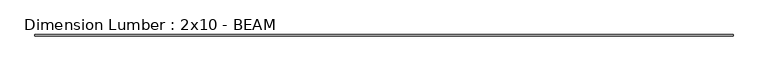
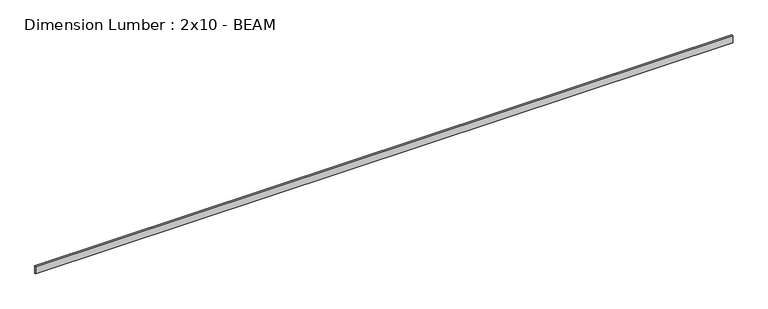
"""IFC4 building model written with IfcOpenShell, lengths in millimetres: beam geometry, Dimension Lumber : 2x10 - BEAM."""

from ifc_helpers import new_model, si_unit, frame, origin, place, context, project, spatial, polyline, outline, extrude, source, transform, mapped, element, save


def dimension_lumber_2x10_beam_73725c05(model_context):
    return source(origin(), model_context, "Body", "SweptSolid", [
        extrude(outline(polyline([(10626.7994141, 19.05), (10626.7994141, -19.05), (-10626.7994141, -19.05), (-10626.7994141, 19.05), (10626.7994141, 19.05)])), frame((0.0, 0.0, -117.475), z_axis=(0.0, 0.0, 1.0), x_axis=(1.0, 0.0, 0.0)), (0.0, 0.0, 1.0), 234.95),
    ])


if __name__ == "__main__":
    model = new_model("IFC4")
    model_context = context("Model", 3, world=origin())
    ifc_project = project(units=[si_unit("LENGTHUNIT", "METRE", prefix="MILLI")], contexts=[model_context])
    site = spatial("IfcSite", under=ifc_project)
    building = spatial("IfcBuilding", under=site)
    placement = place(None, origin())
    dimension_lumber_2x10_beam_shape = dimension_lumber_2x10_beam_73725c05(model_context)
    element("IfcBeam", 1, ObjectType="Dimension Lumber : 2x10 - BEAM", at=placement, inside=building, context=model_context, shape_type="MappedRepresentation", body=[
        mapped(dimension_lumber_2x10_beam_shape, transform((0.0, 0.0, 0.0), x_axis=(1.0, 0.0, 0.0), y_axis=(0.0, 1.0, 0.0), z_axis=(0.0, 0.0, 1.0))),
    ])
    save(model, "model.ifc")

# Revit data of these elements
# Type "Dimension Lumber : 2x10 - BEAM"
#   Assembly Code = "B10"
#   A = 0.0755556 SF
#   Length [instance default] = 5' - 0"
#   b = 0' - 1 1/2"
#   d = 0' - 9 1/4"
#   Structural Material = (3) SISTERED 2X10s AT BEAM
# Element 1 (IfcBeam, "Dimension Lumber : 2x10 - BEAM")
#   Materials on its faces: "(3) SISTERED 2X10s AT BEAM"
# Materials
#   "(3) SISTERED 2X10s AT BEAM": class "Wood", colour RGB 234 198 147, transparency 0, Description = "Pinus Echinata", Cost = 0
